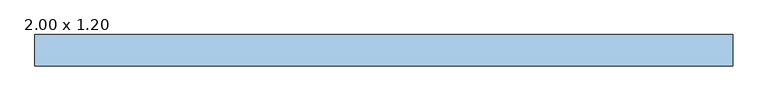
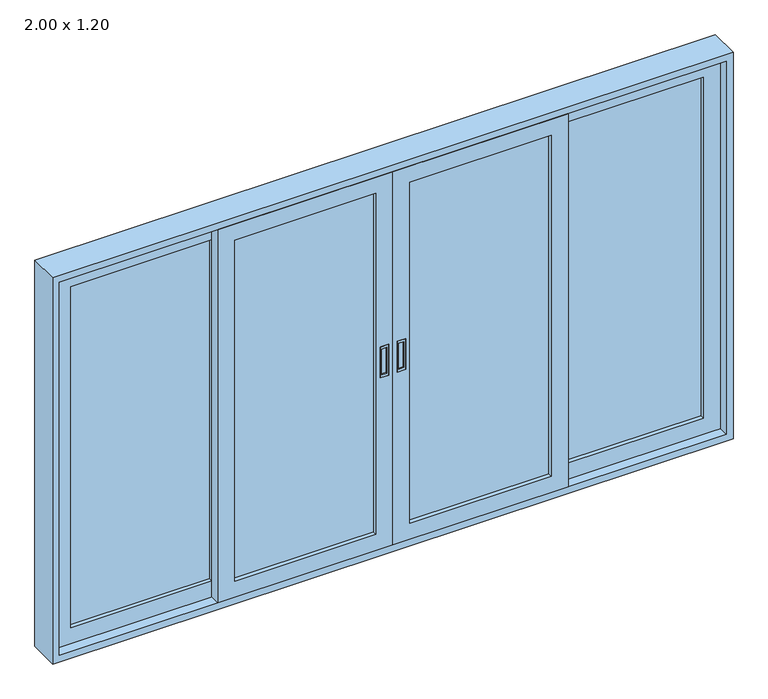
"""IFC4 building model written with IfcOpenShell, lengths in millimetres: window geometry, CC_JANELA CORRER_4 FOLHAS VIDRO : 2.00 x 1.20."""

from ifc_helpers import new_model, si_unit, frame, origin, place, context, project, spatial, polyline, outline, extrude, faceted_brep, source, transform, mapped, element, save


def window_2_00_x_1_20_63c3f2e4(model_context):
    return source(origin(), model_context, "Body", "SolidModel", [
        extrude(outline(polyline([(17.5, -96.0), (17.5, -95.0), (32.5, -95.0), (32.5, -96.0), (17.5, -96.0)])), frame((0.0, 0.0, 1560.0), z_axis=(0.0, 0.0, 1.0), x_axis=(1.0, 0.0, 0.0)), (0.0, 0.0, 1.0), 80.0),
        extrude(outline(polyline([(1552.0, 37.5), (1648.0, 37.5), (1648.0, 12.5), (1552.0, 12.5), (1552.0, 37.5)]), holes=[polyline([(1560.0, 32.5), (1560.0, 17.5), (1640.0, 17.5), (1640.0, 32.5), (1560.0, 32.5)])]), frame((0.0, -100.1, 0.0), z_axis=(0.0, 1.0, 0.0), x_axis=(0.0, 0.0, 1.0)), (0.0, 0.0, 1.0), 5.1),
        faceted_brep([(50.0, -100.0, 2130.0), (50.0, -100.0, 1070.0), (50.0, -70.0, 1070.0), (50.0, -70.0, 2130.0), (0.0, -70.0, 2180.0), (515.0, -70.0, 2180.0), (515.0, -70.0, 1020.0), (0.0, -70.0, 1020.0), (465.0, -70.0, 1070.0), (465.0, -70.0, 2130.0), (465.0, -100.0, 1070.0), (0.0, -100.0, 1020.0), (515.0, -100.0, 1020.0), (515.0, -100.0, 2180.0), (0.0, -100.0, 2180.0), (37.5, -100.0, 1648.0), (37.5, -100.0, 1552.0), (12.5, -100.0, 1552.0), (12.5, -100.0, 1648.0), (465.0, -100.0, 2130.0), (12.5, -95.0, 1552.0), (12.5, -95.0, 1648.0), (37.5, -95.0, 1552.0), (37.5, -95.0, 1648.0)], [[[0, 1, 2, 3]], [[4, 5, 6, 7], [2, 8, 9, 3]], [[1, 10, 8, 2]], [[11, 12, 13, 14], [15, 16, 17, 18], [0, 19, 10, 1]], [[4, 7, 11, 14]], [[7, 6, 12, 11]], [[10, 19, 9, 8]], [[6, 5, 13, 12]], [[18, 17, 20, 21]], [[20, 17, 16, 22]], [[23, 22, 16, 15]], [[21, 20, 22, 23]], [[3, 9, 19, 0]], [[14, 13, 5, 4]], [[21, 23, 15, 18]]]),
        extrude(outline(polyline([(50.0, -82.5), (465.0, -82.5), (465.0, -87.5), (50.0, -87.5), (50.0, -82.5)])), frame((0.0, 0.0, 1070.0), z_axis=(0.0, 0.0, 1.0), x_axis=(1.0, 0.0, 0.0)), (0.0, 0.0, 1.0), 1060.0),
        extrude(outline(polyline([(-17.5, -96.0), (-32.5, -96.0), (-32.5, -95.0), (-17.5, -95.0), (-17.5, -96.0)])), frame((0.0, 0.0, 1560.0), z_axis=(0.0, 0.0, 1.0), x_axis=(1.0, 0.0, 0.0)), (0.0, 0.0, 1.0), 80.0),
        extrude(outline(polyline([(1552.0, -37.5), (1552.0, -12.5), (1648.0, -12.5), (1648.0, -37.5), (1552.0, -37.5)]), holes=[polyline([(1560.0, -32.5), (1640.0, -32.5), (1640.0, -17.5), (1560.0, -17.5), (1560.0, -32.5)])]), frame((0.0, -100.1, 0.0), z_axis=(0.0, 1.0, 0.0), x_axis=(0.0, 0.0, 1.0)), (0.0, 0.0, 1.0), 5.1),
        faceted_brep([(-50.0, -100.0, 2130.0), (-50.0, -70.0, 2130.0), (-50.0, -70.0, 1070.0), (-50.0, -100.0, 1070.0), (0.0, -70.0, 2180.0), (0.0, -70.0, 1020.0), (-515.0, -70.0, 1020.0), (-515.0, -70.0, 2180.0), (-465.0, -70.0, 2130.0), (-465.0, -70.0, 1070.0), (-465.0, -100.0, 1070.0), (0.0, -100.0, 1020.0), (0.0, -100.0, 2180.0), (-515.0, -100.0, 2180.0), (-515.0, -100.0, 1020.0), (-465.0, -100.0, 2130.0), (-37.5, -100.0, 1648.0), (-12.5, -100.0, 1648.0), (-12.5, -100.0, 1552.0), (-37.5, -100.0, 1552.0), (-12.5, -95.0, 1648.0), (-12.5, -95.0, 1552.0), (-37.5, -95.0, 1552.0), (-37.5, -95.0, 1648.0)], [[[0, 1, 2, 3]], [[4, 5, 6, 7], [2, 1, 8, 9]], [[3, 2, 9, 10]], [[11, 12, 13, 14], [0, 3, 10, 15], [16, 17, 18, 19]], [[4, 12, 11, 5]], [[5, 11, 14, 6]], [[10, 9, 8, 15]], [[6, 14, 13, 7]], [[17, 20, 21, 18]], [[21, 22, 19, 18]], [[23, 16, 19, 22]], [[20, 23, 22, 21]], [[1, 0, 15, 8]], [[12, 4, 7, 13]], [[20, 17, 16, 23]]]),
        extrude(outline(polyline([(-50.0, -82.5), (-50.0, -87.5), (-465.0, -87.5), (-465.0, -82.5), (-50.0, -82.5)])), frame((0.0, 0.0, 1070.0), z_axis=(0.0, 0.0, 1.0), x_axis=(1.0, 0.0, 0.0)), (0.0, 0.0, 1.0), 1060.0),
        extrude(outline(polyline([(930.0, -52.5), (930.0, -57.5), (515.0, -57.5), (515.0, -52.5), (930.0, -52.5)])), frame((0.0, 0.0, 1070.0), z_axis=(0.0, 0.0, 1.0), x_axis=(1.0, 0.0, 0.0)), (0.0, 0.0, 1.0), 1060.0),
        extrude(outline(polyline([(2180.0, 980.0), (2180.0, 465.0), (1020.0, 465.0), (1020.0, 980.0), (2180.0, 980.0)]), holes=[polyline([(1070.0, 930.0), (1070.0, 515.0), (2130.0, 515.0), (2130.0, 930.0), (1070.0, 930.0)])]), frame((0.0, -70.0, 0.0), z_axis=(0.0, 1.0, 0.0), x_axis=(0.0, 0.0, 1.0)), (0.0, 0.0, 1.0), 30.0),
        extrude(outline(polyline([(-515.0, -52.5), (-515.0, -57.5), (-930.0, -57.5), (-930.0, -52.5), (-515.0, -52.5)])), frame((0.0, 0.0, 1070.0), z_axis=(0.0, 0.0, 1.0), x_axis=(1.0, 0.0, 0.0)), (0.0, 0.0, 1.0), 1060.0),
        extrude(outline(polyline([(2180.0, -465.0), (2180.0, -980.0), (1020.0, -980.0), (1020.0, -465.0), (2180.0, -465.0)]), holes=[polyline([(1070.0, -515.0), (1070.0, -930.0), (2130.0, -930.0), (2130.0, -515.0), (1070.0, -515.0)])]), frame((0.0, -70.0, 0.0), z_axis=(0.0, 1.0, 0.0), x_axis=(0.0, 0.0, 1.0)), (0.0, 0.0, 1.0), 30.0),
        extrude(outline(polyline([(2200.0, 1000.0), (2200.0, -1000.0), (1000.0, -1000.0), (1000.0, 1000.0), (2200.0, 1000.0)]), holes=[polyline([(2180.0, 980.0), (1020.0, 980.0), (1020.0, -980.0), (2180.0, -980.0), (2180.0, 980.0)])]), frame((0.0, -100.0, 0.0), z_axis=(0.0, 1.0, 0.0), x_axis=(0.0, 0.0, 1.0)), (0.0, 0.0, 1.0), 90.0),
    ])


if __name__ == "__main__":
    model = new_model("IFC4")
    model_context = context("Model", 3, world=origin())
    ifc_project = project(units=[si_unit("LENGTHUNIT", "METRE", prefix="MILLI")], contexts=[model_context])
    site = spatial("IfcSite", under=ifc_project)
    building = spatial("IfcBuilding", under=site)
    placement = place(None, origin())
    window_2_00_x_1_20_shape = window_2_00_x_1_20_63c3f2e4(model_context)
    element("IfcWindow", 1, ObjectType="CC_JANELA CORRER_4 FOLHAS VIDRO : 2.00 x 1.20", at=placement, inside=building, context=model_context, shape_type="MappedRepresentation", body=[
        mapped(window_2_00_x_1_20_shape, transform((0.0, 0.0, 0.0), x_axis=(1.0, 0.0, 0.0), y_axis=(0.0, 1.0, 0.0), z_axis=(0.0, 0.0, 1.0))),
    ])
    save(model, "model.ifc")

# Revit data of these elements
# Type "CC_JANELA CORRER_4 FOLHAS VIDRO : 2.00 x 1.20"
#   Type Mark = "J5"
#   Site = "www.construir.arq.br"
#   Emprea = "Cursos Construir"
#   Criado Por = "Roberto Netto"
#   Analytic Construction = "<Nenhum>"
#   Rough Width = 2.00 m
#   Largura Moldura Folha [instance default] = 0.05 m
#   Largura Guarnição Interna [instance default] = 0.10 m
#   Largura Moldura Externa [instance default] = 0.10 m
#   Largura Folha [instance default] = 0.515 m
#   Interna [instance default] = 0.00 m
#   Externa [instance default] = 0.00 m
#   Extensão Frontal Peitoril/Pingadeira [instance default] = 0.03 m
#   Extensão Exterior Esquerda Peitoril/Pingadeira [instance default] = 0.025 m
#   Extensão Exterior Direita Peitoril/Pingadeira [instance default] = 0.025 m
#   Extensão Caixilho [instance default] = 0.03 m
#   Espessura Peitoril/Pingadeira [instance default] = 0.02 m
#   Espessura Guarnição Interna [instance default] = 0.005 m
#   Espessura Moldura Externa [instance default] = 0.01 m
#   Espessura Folha [instance default] = 0.03 m
#   Cálculo Porcentagem [instance default] = 0.00 m
#   Cálculo Abertura [instance default] = 0.00 m
#   Espessura Caixilho [instance default] = 0.02 m
#   Rough Height = 1.20 m
#   Altura Folha [instance default] = 1.16 m
#   Altura Corte [instance default] = 0.02 m
#   Height = 1.20 m
#   Width = 2.00 m
#   ----PEITORIL/PINGADEIRA--- [instance default] = 0.00 m
#   ----MOLDURA---- [instance default] = 0.00 m
#   ----GUARNIÇÃO---- [instance default] = 0.00 m
#   ----EXTENSÃO---- [instance default] = 0.00 m
#   ----CAIXILHO---- [instance default] = 0.00 m
#   -----FOLHA---- [instance default] = 0.00 m
#   Puxador [instance default] = yes
#   Peitoril/Pingadeira Vazio [instance default] = no
#   Peitoril/Pingadeira Família [instance default] = yes
#   Guarnição Interna [instance default] = yes
#   Moldura Externa Sem Peitoril [instance default] = no
#   Moldura Externa Com Peitoril [instance default] = yes
#   Moldura Externa [instance default] = yes
#   Material Vidro Folha = .VIDRO
#   Material Puxador = .ALUMÍNIO COM PINTURA ELETROSTÁTICA BRANCA
#   Material Peitoril/Pingadeira = .GRANITO BRANCO ITAÚNAS
#   Material Moldura Folha = .ALUMÍNIO COM PINTURA ELETROSTÁTICA BRANCA
#   Material Moldura Externa = .PINTURA ACRÍLICA BRANCA
#   Material Caixilho = .ALUMÍNIO COM PINTURA ELETROSTÁTICA BRANCA
#   Material Guarnição = .ALUMÍNIO COM PINTURA ELETROSTÁTICA BRANCA
#   Wall Closure = (empty or 0)
# Element 1 (IfcWindow, "CC_JANELA CORRER_4 FOLHAS VIDRO : 2.00 x 1.20")
#   Guarnição Interna = no
#   Moldura Externa Com Peitoril = no
#   Moldura Externa = no
#   Materials on its faces: ".ALUMÍNIO COM PINTURA ELETROSTÁTICA BRANCA", ".VIDRO"
# Materials
#   ".VIDRO": class "Genérico", colour RGB 198 236 255, transparency 0.95, Cost = 0
#   ".ALUMÍNIO COM PINTURA ELETROSTÁTICA BRANCA": class "CC_METAIS", colour RGB 241 241 241, transparency 0, Cost = 0
#   ".GRANITO BRANCO ITAÚNAS": class ".CC_PEDRA REVEST.", colour RGB 202 195 174, transparency 0, Description = "Granito branco Itaúnas", Uso = "Pedra", Cost = 0
#   ".PINTURA ACRÍLICA BRANCA": class ".CC_PINTURA", colour RGB 250 250 250, transparency 0, Keynote = "09910.A1", Description = "Tinta acrílica na cor branca", Cost = 0
